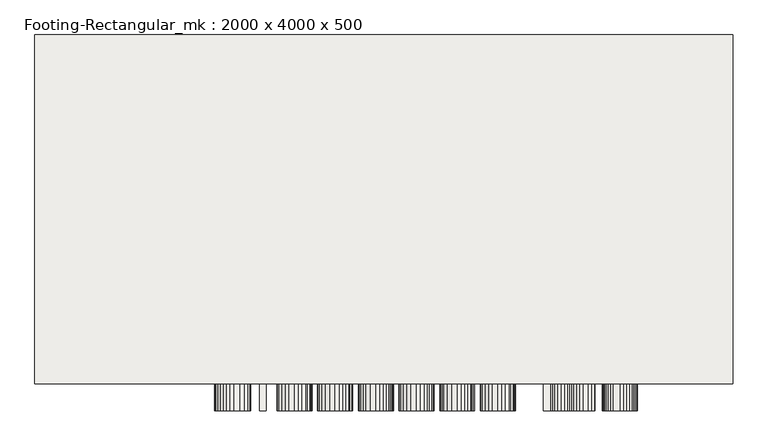
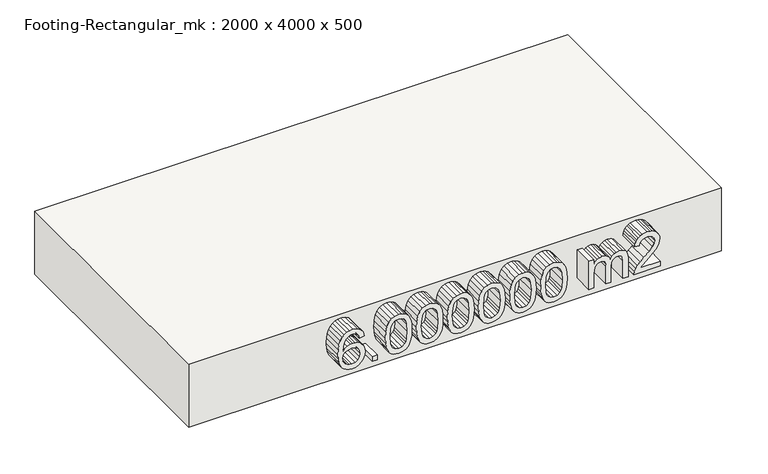
"""IFC4 building model written with IfcOpenShell, lengths in millimetres: slab geometry, Footing-Rectangular_mk : 2000 x 4000 x 500."""

from ifc_helpers import new_model, si_unit, frame, origin, place, context, project, spatial, polyline, outline, extrude, source, transform, mapped, element, save


def footing_rectangular_mk_2000_x_4000_x_500_7c447ffd(model_context):
    return source(origin(), model_context, "Body", "SweptSolid", [
        extrude(outline(polyline([(2000.0, 1085.6), (2000.0, -914.4), (-2000.0, -914.4), (-2000.0, 1085.6), (2000.0, 1085.6)])), frame((0.0, 0.0, -500.0), z_axis=(0.0, 0.0, 1.0), x_axis=(1.0, 0.0, 0.0)), (0.0, 0.0, 1.0), 500.0),
        extrude(outline(polyline([(-113.8433338, -768.5560264), (-80.0293968, -777.9250337), (-54.4319304, -796.6630483), (-38.3150072, -823.4130513), (-32.9426994, -856.8180237), (-35.1130002, -880.170832), (-41.6239026, -901.0047902), (-52.4754066, -919.3198982), (-67.6675122, -935.116156), (-90.5927666, -949.6901673), (-119.5130704, -960.1001754), (-154.4284234, -966.3461803), (-195.3388258, -968.4281819), (-231.829622, -966.5529863), (-262.7808068, -960.9273993), (-288.1923801, -951.551421), (-308.064342, -938.4250514), (-323.0287287, -922.3243938), (-333.7175763, -904.0255515), (-340.1308848, -883.5285244), (-342.2686543, -860.8333125), (-339.0434108, -834.417917), (-329.36768, -810.9396308), (-313.6225428, -791.2907406), (-292.1890797, -776.3635325), (-266.9169261, -766.9387573), (-239.6557174, -763.7971656), (-219.1563666, -765.4655553), (-200.6367763, -770.4707244), (-184.0969465, -778.8126728), (-169.5368771, -790.4914006), (-157.6629616, -804.5449116), (-149.1815934, -820.0112093), (-144.0927725, -836.8902939), (-142.3964989, -855.1821653), (-144.8781704, -876.4762086), (-152.3231852, -896.785019), (-164.8802574, -915.0861851), (-182.6981016, -930.3572952), (-143.2051334, -927.4294804), (-114.847156, -919.5383225), (-94.7985958, -907.8549473), (-80.2338791, -893.5504808), (-73.3186594, -876.8944679), (-71.0135862, -859.1974541), (-74.9731071, -838.32167), (-86.8516699, -821.0522101), (-99.734055, -812.7613823), (-118.6021946, -806.6269132), (-113.8433338, -768.5560264)]), holes=[polyline([(-239.0608598, -930.3572952), (-215.3316181, -925.6263183), (-196.6400768, -911.4333876), (-184.5105584, -890.4553623), (-180.4673856, -865.3691017), (-184.5105584, -838.7956971), (-196.6400768, -818.7099583), (-215.7963506, -806.0785288), (-240.9197898, -801.8680524), (-267.0935244, -806.1342967), (-287.1699686, -818.9330299), (-299.9408179, -838.6841613), (-304.1977676, -863.8076005), (-302.1436499, -882.2388917), (-295.9812969, -898.1234487), (-285.8873069, -911.2846732), (-272.0382783, -921.5459669), (-255.9306497, -928.1544631), (-239.0608598, -930.3572952)])]), frame((0.0, -1066.8, 0.0), z_axis=(0.0, 1.0, 0.0), x_axis=(0.0, 0.0, 1.0)), (0.0, 0.0, 1.0), 152.4),
        extrude(outline(polyline([(-673.3788095, -1066.8), (-711.4496963, -1066.8), (-711.4496963, -914.4), (-673.3788095, -914.4), (-673.3788095, -1066.8)])), frame((0.0, 0.0, -337.5097935), z_axis=(0.0, 0.0, 1.0), x_axis=(1.0, 0.0, 0.0)), (0.0, 0.0, 1.0), 38.0708868),
        extrude(outline(polyline([(-187.6800341, -611.5136186), (-227.540141, -609.6175099), (-261.7583953, -603.9291841), (-290.334797, -594.448641), (-313.2693461, -581.1758807), (-325.9565434, -567.3454413), (-335.0188273, -551.1355716), (-340.4561976, -532.5462714), (-342.2686543, -511.5775408), (-338.0953565, -480.8029544), (-325.5754628, -455.8468189), (-304.5695536, -436.5418307), (-274.9382091, -422.720686), (-236.1516343, -414.4112688), (-187.6800341, -411.6414631), (-147.2947795, -413.370268), (-116.1112284, -418.5566827), (-91.5547629, -426.4757246), (-71.0507648, -436.4024109), (-54.7386539, -449.5450461), (-42.7578499, -467.1119348), (-35.3964871, -488.117844), (-32.9426994, -511.5775408), (-37.0881134, -542.1848236), (-49.5243552, -567.0851911), (-70.4466125, -586.4180633), (-100.0500731, -600.3228599), (-138.9295944, -608.7159289), (-187.6800341, -611.5136186)]), holes=[polyline([(-187.6056769, -573.4427318), (-128.4917023, -568.8325854), (-107.1883643, -563.0699023), (-91.3874592, -555.002146), (-76.1070544, -535.8551668), (-71.0135862, -512.023684), (-76.7948585, -486.8537716), (-94.1386756, -466.9632204), (-108.6522717, -459.4159645), (-129.0679706, -454.0250675), (-187.6056769, -449.7123498), (-247.3981609, -454.1737819), (-267.8765987, -459.7505719), (-282.0765004, -467.558078), (-298.6674508, -487.4858078), (-304.1977676, -511.5775408), (-298.6860401, -535.6692738), (-282.1508576, -555.5970036), (-267.9741925, -563.4045097), (-247.4911074, -568.9812998), (-187.6056769, -573.4427318)])]), frame((0.0, -1066.8, 0.0), z_axis=(0.0, 1.0, 0.0), x_axis=(0.0, 0.0, 1.0)), (0.0, 0.0, 1.0), 152.4),
        extrude(outline(polyline([(-187.6800341, -378.3294372), (-227.540141, -376.4333285), (-261.7583953, -370.7450027), (-290.334797, -361.2644596), (-313.2693461, -347.9916993), (-325.9565434, -334.1612599), (-335.0188273, -317.9513902), (-340.4561976, -299.36209), (-342.2686543, -278.3933594), (-338.0953565, -247.618773), (-325.5754628, -222.6626375), (-304.5695536, -203.3576493), (-274.9382091, -189.5365046), (-236.1516343, -181.2270874), (-187.6800341, -178.4572817), (-147.2947795, -180.1860866), (-116.1112284, -185.3725013), (-91.5547629, -193.2915432), (-71.0507648, -203.2182295), (-54.7386539, -216.3608647), (-42.7578499, -233.9277534), (-35.3964871, -254.9336626), (-32.9426994, -278.3933594), (-37.0881134, -309.0006422), (-49.5243552, -333.9010097), (-70.4466125, -353.2338819), (-100.0500731, -367.1386785), (-138.9295944, -375.5317475), (-187.6800341, -378.3294372)]), holes=[polyline([(-187.6056769, -340.2585504), (-128.4917023, -335.648404), (-107.1883643, -329.8857209), (-91.3874592, -321.8179646), (-76.1070544, -302.6709855), (-71.0135862, -278.8395026), (-76.7948585, -253.6695902), (-94.1386756, -233.779039), (-108.6522717, -226.2317831), (-129.0679706, -220.8408861), (-187.6056769, -216.5281684), (-247.3981609, -220.9896005), (-267.8765987, -226.5663905), (-282.0765004, -234.3738966), (-298.6674508, -254.3016264), (-304.1977676, -278.3933594), (-298.6860401, -302.4850924), (-282.1508576, -322.4128222), (-267.9741925, -330.2203283), (-247.4911074, -335.7971184), (-187.6056769, -340.2585504)])]), frame((0.0, -1066.8, 0.0), z_axis=(0.0, 1.0, 0.0), x_axis=(0.0, 0.0, 1.0)), (0.0, 0.0, 1.0), 152.4),
        extrude(outline(polyline([(-187.6800341, -145.1452558), (-227.540141, -143.2491471), (-261.7583953, -137.5608213), (-290.334797, -128.0802782), (-313.2693461, -114.8075179), (-325.9565434, -100.9770786), (-335.0188273, -84.7672088), (-340.4561976, -66.1779086), (-342.2686543, -45.209178), (-338.0953565, -14.4345916), (-325.5754628, 10.5215439), (-304.5695536, 29.8265321), (-274.9382091, 43.6476768), (-236.1516343, 51.957094), (-187.6800341, 54.7268997), (-147.2947795, 52.9980948), (-116.1112284, 47.8116801), (-91.5547629, 39.8926382), (-71.0507648, 29.9659519), (-54.7386539, 16.8233167), (-42.7578499, -0.743572), (-35.3964871, -21.7494812), (-32.9426994, -45.209178), (-37.0881134, -75.8164608), (-49.5243552, -100.7168283), (-70.4466125, -120.0497005), (-100.0500731, -133.9544971), (-138.9295944, -142.3475661), (-187.6800341, -145.1452558)]), holes=[polyline([(-187.6056769, -107.074369), (-128.4917023, -102.4642226), (-107.1883643, -96.7015395), (-91.3874592, -88.6337832), (-76.1070544, -69.4868041), (-71.0135862, -45.6553212), (-76.7948585, -20.4854088), (-94.1386756, -0.5948576), (-108.6522717, 6.9523983), (-129.0679706, 12.3432953), (-187.6056769, 16.656013), (-247.3981609, 12.1945809), (-267.8765987, 6.6177909), (-282.0765004, -1.1897152), (-298.6674508, -21.117445), (-304.1977676, -45.209178), (-298.6860401, -69.3009111), (-282.1508576, -89.2286408), (-267.9741925, -97.0361469), (-247.4911074, -102.612937), (-187.6056769, -107.074369)])]), frame((0.0, -1066.8, 0.0), z_axis=(0.0, 1.0, 0.0), x_axis=(0.0, 0.0, 1.0)), (0.0, 0.0, 1.0), 152.4),
        extrude(outline(polyline([(-187.6800341, 88.0389256), (-227.540141, 89.9350342), (-261.7583953, 95.6233601), (-290.334797, 105.1039032), (-313.2693461, 118.3766635), (-325.9565434, 132.2071028), (-335.0188273, 148.4169726), (-340.4561976, 167.0062728), (-342.2686543, 187.9750034), (-338.0953565, 218.7495898), (-325.5754628, 243.7057253), (-304.5695536, 263.0107135), (-274.9382091, 276.8318582), (-236.1516343, 285.1412754), (-187.6800341, 287.9110811), (-147.2947795, 286.1822762), (-116.1112284, 280.9958614), (-91.5547629, 273.0768196), (-71.0507648, 263.1501333), (-54.7386539, 250.0074981), (-42.7578499, 232.4406094), (-35.3964871, 211.4347002), (-32.9426994, 187.9750034), (-37.0881134, 157.3677206), (-49.5243552, 132.467353), (-70.4466125, 113.1344809), (-100.0500731, 99.2296843), (-138.9295944, 90.8366153), (-187.6800341, 88.0389256)]), holes=[polyline([(-187.6056769, 126.1098124), (-128.4917023, 130.7199588), (-107.1883643, 136.4826419), (-91.3874592, 144.5503982), (-76.1070544, 163.6973773), (-71.0135862, 187.5288602), (-76.7948585, 212.6987726), (-94.1386756, 232.5893238), (-108.6522717, 240.1365797), (-129.0679706, 245.5274767), (-187.6056769, 249.8401944), (-247.3981609, 245.3787623), (-267.8765987, 239.8019723), (-282.0765004, 231.9944662), (-298.6674508, 212.0667364), (-304.1977676, 187.9750034), (-298.6860401, 163.8832703), (-282.1508576, 143.9555406), (-267.9741925, 136.1480345), (-247.4911074, 130.5712444), (-187.6056769, 126.1098124)])]), frame((0.0, -1066.8, 0.0), z_axis=(0.0, 1.0, 0.0), x_axis=(0.0, 0.0, 1.0)), (0.0, 0.0, 1.0), 152.4),
        extrude(outline(polyline([(-187.6800341, 321.223107), (-227.540141, 323.1192156), (-261.7583953, 328.8075415), (-290.334797, 338.2880846), (-313.2693461, 351.5608449), (-325.9565434, 365.3912842), (-335.0188273, 381.601154), (-340.4561976, 400.1904542), (-342.2686543, 421.1591848), (-338.0953565, 451.9337712), (-325.5754628, 476.8899067), (-304.5695536, 496.1948949), (-274.9382091, 510.0160396), (-236.1516343, 518.3254568), (-187.6800341, 521.0952625), (-147.2947795, 519.3664576), (-116.1112284, 514.1800428), (-91.5547629, 506.261001), (-71.0507648, 496.3343147), (-54.7386539, 483.1916795), (-42.7578499, 465.6247908), (-35.3964871, 444.6188816), (-32.9426994, 421.1591848), (-37.0881134, 390.551902), (-49.5243552, 365.6515344), (-70.4466125, 346.3186623), (-100.0500731, 332.4138657), (-138.9295944, 324.0207967), (-187.6800341, 321.223107)]), holes=[polyline([(-187.6056769, 359.2939938), (-128.4917023, 363.9041402), (-107.1883643, 369.6668233), (-91.3874592, 377.7345796), (-76.1070544, 396.8815587), (-71.0135862, 420.7130416), (-76.7948585, 445.882954), (-94.1386756, 465.7735052), (-108.6522717, 473.3207611), (-129.0679706, 478.7116581), (-187.6056769, 483.0243757), (-247.3981609, 478.5629437), (-267.8765987, 472.9861537), (-282.0765004, 465.1786476), (-298.6674508, 445.2509178), (-304.1977676, 421.1591848), (-298.6860401, 397.0674517), (-282.1508576, 377.139722), (-267.9741925, 369.3322159), (-247.4911074, 363.7554258), (-187.6056769, 359.2939938)])]), frame((0.0, -1066.8, 0.0), z_axis=(0.0, 1.0, 0.0), x_axis=(0.0, 0.0, 1.0)), (0.0, 0.0, 1.0), 152.4),
        extrude(outline(polyline([(-187.6800341, 554.4072884), (-227.540141, 556.303397), (-261.7583953, 561.9917229), (-290.334797, 571.472266), (-313.2693461, 584.7450263), (-325.9565434, 598.5754656), (-335.0188273, 614.7853354), (-340.4561976, 633.3746356), (-342.2686543, 654.3433662), (-338.0953565, 685.1179526), (-325.5754628, 710.0740881), (-304.5695536, 729.3790763), (-274.9382091, 743.200221), (-236.1516343, 751.5096382), (-187.6800341, 754.2794439), (-147.2947795, 752.550639), (-116.1112284, 747.3642242), (-91.5547629, 739.4451824), (-71.0507648, 729.5184961), (-54.7386539, 716.3758608), (-42.7578499, 698.8089722), (-35.3964871, 677.803063), (-32.9426994, 654.3433662), (-37.0881134, 623.7360834), (-49.5243552, 598.8357158), (-70.4466125, 579.5028437), (-100.0500731, 565.5980471), (-138.9295944, 557.2049781), (-187.6800341, 554.4072884)]), holes=[polyline([(-187.6056769, 592.4781752), (-128.4917023, 597.0883216), (-107.1883643, 602.8510047), (-91.3874592, 610.918761), (-76.1070544, 630.0657401), (-71.0135862, 653.897223), (-76.7948585, 679.0671354), (-94.1386756, 698.9576866), (-108.6522717, 706.5049425), (-129.0679706, 711.8958395), (-187.6056769, 716.2085571), (-247.3981609, 711.7471251), (-267.8765987, 706.1703351), (-282.0765004, 698.362829), (-298.6674508, 678.4350992), (-304.1977676, 654.3433662), (-298.6860401, 630.2516331), (-282.1508576, 610.3239033), (-267.9741925, 602.5163973), (-247.4911074, 596.9396072), (-187.6056769, 592.4781752)])]), frame((0.0, -1066.8, 0.0), z_axis=(0.0, 1.0, 0.0), x_axis=(0.0, 0.0, 1.0)), (0.0, 0.0, 1.0), 152.4),
        extrude(outline(polyline([(-337.5097935, 916.0807126), (-337.5097935, 954.1515994), (-224.70992, 954.1515994), (-198.5175961, 955.6015648), (-179.2776704, 959.951461), (-165.4100525, 967.5358955), (-155.3346518, 978.6894756), (-149.2001827, 992.2038968), (-147.1553597, 1006.8708547), (-150.2225942, 1024.1310199), (-159.4242978, 1035.7586272), (-174.7790598, 1042.3671234), (-196.3054694, 1044.5699554), (-337.5097935, 1044.5699554), (-337.5097935, 1082.6408422), (-211.2512667, 1082.6408422), (-182.2333691, 1086.3679969), (-162.3985859, 1097.5494609), (-150.9661662, 1114.3634829), (-147.1553597, 1134.9883115), (-148.6425037, 1146.6716866), (-153.1039358, 1156.7377927), (-159.9912715, 1164.5638881), (-168.7561265, 1169.5272312), (-200.5438298, 1173.0591982), (-337.5097935, 1173.0591982), (-337.5097935, 1211.130085), (-184.1852457, 1211.130085), (-150.8639251, 1206.7708941), (-127.4878801, 1193.6933214), (-113.6853247, 1172.5294032), (-109.084473, 1143.9111756), (-111.8496314, 1124.1786334), (-120.1451066, 1106.3979678), (-133.9708986, 1090.5691787), (-153.3270074, 1076.6922661), (-134.6912339, 1068.4014383), (-120.7213749, 1055.7235355), (-111.9936984, 1038.7515045), (-109.084473, 1017.5782916), (-111.9379305, 997.8178655), (-120.4983033, 980.325334), (-133.7431796, 965.6026083), (-150.6501481, 954.1515994), (-113.8433338, 954.1515994), (-113.8433338, 916.0807126), (-337.5097935, 916.0807126)])), frame((0.0, -1066.8, 0.0), z_axis=(0.0, 1.0, 0.0), x_axis=(0.0, 0.0, 1.0)), (0.0, 0.0, 1.0), 152.4),
        extrude(outline(polyline([(-299.4389067, 1453.8319881), (-299.4389067, 1304.2996575), (-280.068856, 1321.4761708), (-243.4479346, 1365.2725621), (-214.1233136, 1398.3150431), (-191.2863583, 1419.8135688), (-172.1579684, 1433.300106), (-153.9590436, 1442.306622), (-136.0668422, 1447.3815009), (-117.8586226, 1449.0731272), (-100.5241002, 1447.504655), (-84.6581325, 1442.7992384), (-70.2607195, 1434.9568774), (-57.3318613, 1423.977572), (-46.661603, 1410.3074654), (-39.0399899, 1394.3927008), (-34.4670221, 1376.2332782), (-32.9426994, 1355.8291976), (-38.426543, 1317.5445339), (-45.2813474, 1301.6437112), (-54.8780736, 1287.9038947), (-67.0865965, 1276.5853346), (-81.776791, 1267.948281), (-98.948657, 1261.9927339), (-118.6021946, 1258.7186935), (-123.3610555, 1296.7895802), (-101.4814492, 1300.9071102), (-84.9183827, 1312.813557), (-74.4897853, 1331.2634374), (-71.0135862, 1355.0112684), (-74.5734372, 1377.625152), (-85.2529901, 1395.4987641), (-101.1003685, 1407.1263714), (-120.1636959, 1411.0022405), (-141.4298553, 1406.8940051), (-163.2908723, 1394.5692991), (-190.2267682, 1369.9198871), (-226.7175645, 1328.8375337), (-250.0192522, 1301.04653), (-270.8485631, 1281.1745681), (-290.7484089, 1267.4370752), (-311.2617017, 1258.0494786), (-337.5097935, 1253.9598326), (-337.5097935, 1453.8319881), (-299.4389067, 1453.8319881)])), frame((0.0, -1066.8, 0.0), z_axis=(0.0, 1.0, 0.0), x_axis=(0.0, 0.0, 1.0)), (0.0, 0.0, 1.0), 152.4),
    ])


if __name__ == "__main__":
    model = new_model("IFC4")
    model_context = context("Model", 3, world=origin())
    ifc_project = project(units=[si_unit("LENGTHUNIT", "METRE", prefix="MILLI")], contexts=[model_context])
    site = spatial("IfcSite", under=ifc_project)
    building = spatial("IfcBuilding", under=site)
    placement = place(None, origin())
    footing_rectangular_mk_2000_x_4000_x_500_shape = footing_rectangular_mk_2000_x_4000_x_500_7c447ffd(model_context)
    element("IfcSlab", 1, ObjectType="Footing-Rectangular_mk : 2000 x 4000 x 500", at=placement, inside=building, context=model_context, shape_type="MappedRepresentation", body=[
        mapped(footing_rectangular_mk_2000_x_4000_x_500_shape, transform((0.0, 0.0, 0.0), x_axis=(1.0, 0.0, 0.0), y_axis=(0.0, 1.0, 0.0), z_axis=(0.0, 0.0, 1.0))),
    ])
    save(model, "model.ifc")

# Revit data of these elements
# Type "Footing-Rectangular_mk : 2000 x 4000 x 500"
#   ModelText [instance default] = "ModelText"
#   Assembly Code = "A1010100"
#   Width = 4000 mm
#   Length = 2000 mm
#   Foundation Thickness = 500 mm
#   Structural Material [instance default] = Concrete, Cast-in-Place gray
# Element 1 (IfcSlab, "Footing-Rectangular_mk : 2000 x 4000 x 500")
#   ModelText = "6.000000 m2"
#   Materials on its faces: "Concrete, Cast-in-Place gray"
# Materials
#   "Concrete, Cast-in-Place gray": class "Concrete", colour RGB 192 192 192, transparency 0, Description = "Cast-in-place concrete", Cost = 0
